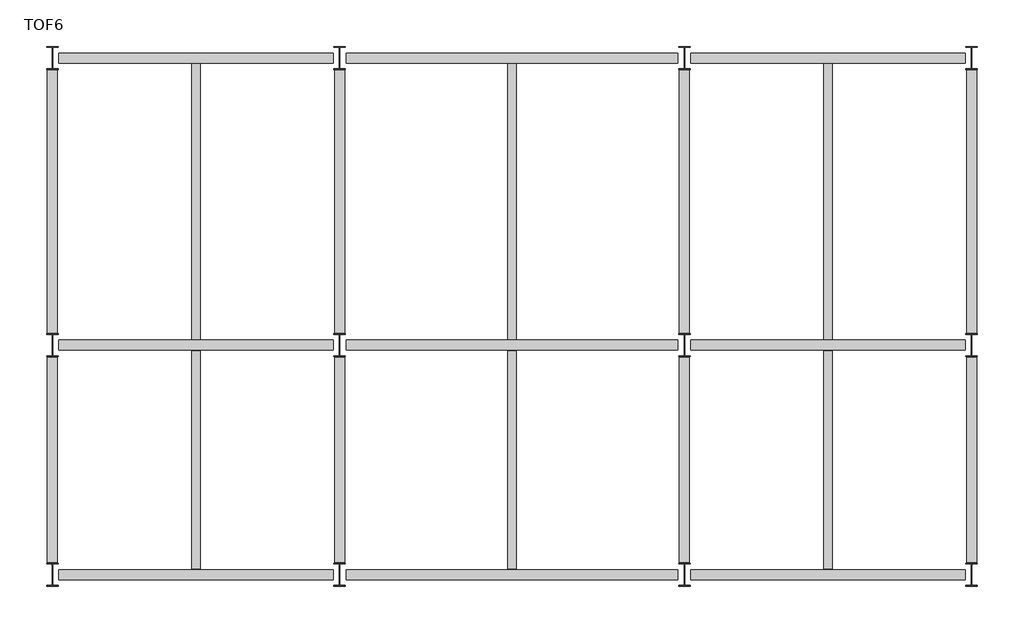
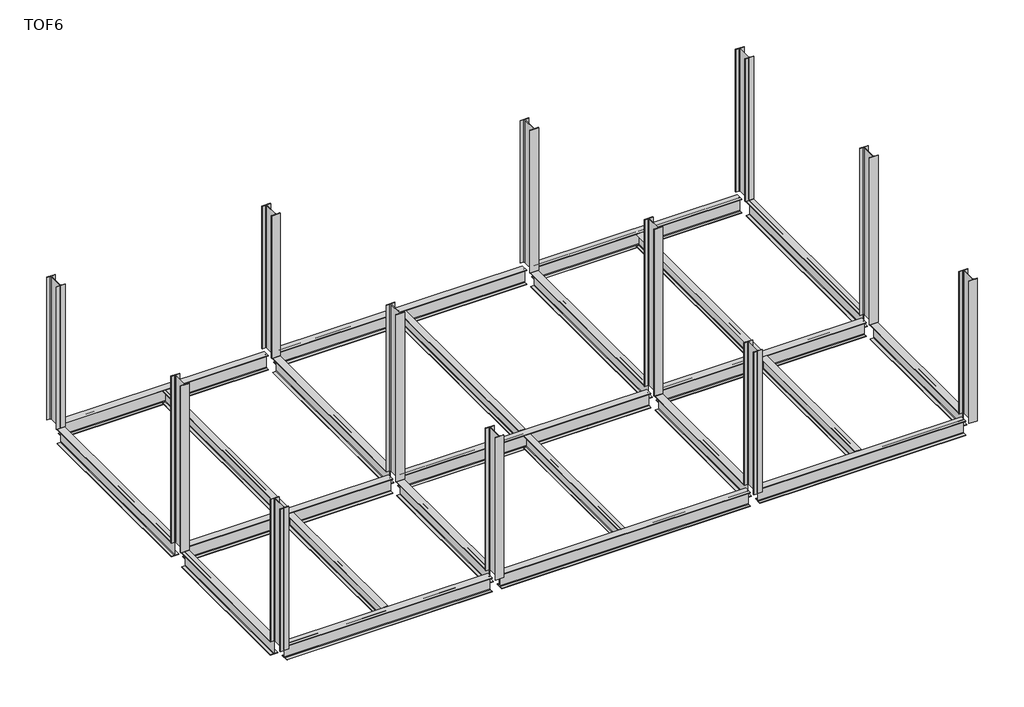
# One storey: 23 beams, 12 columns.
"""IFC4 building model written with IfcOpenShell, lengths in millimetres."""

import ifcopenshell
import ifcopenshell.guid

model = None  # the IFC model being written
_history = None  # IfcOwnerHistory: only IFC2X3 demands one
_inside = {}  # id of a spatial element -> (the spatial element, [elements in it])
_under = {}  # id of a project, library or spatial element -> (it, [spatial elements below it])
_declared = {}  # id of a project -> (the project, [libraries it declares])
_typed = {}  # id of a type object -> (the type object, [elements of that type])
_made_of = {}  # id of a material, layer set ... -> (it, [elements and type objects made of it])


def new_model(schema):
    """Start an empty IFC model of exactly this schema.

    Asked for "IFC4X3", IfcOpenShell would pick the latest addendum, in which some entities
    have other attributes; the version numbers below select the first issue.
    IFC2X3 requires an IfcOwnerHistory on every rooted entity: one is made here for all.
    """
    global model, _history
    if schema == "IFC4X3":
        model = ifcopenshell.file(schema_version=(4, 3, 0, 0))
    else:
        model = ifcopenshell.file(schema=schema)
    _inside.clear()
    _under.clear()
    _declared.clear()
    _typed.clear()
    _made_of.clear()
    _history = None
    if model.schema == "IFC2X3":
        org = make("IfcOrganization", Name="unknown")
        user = make(
            "IfcPersonAndOrganization",
            ThePerson=make("IfcPerson", FamilyName="unknown"),
            TheOrganization=org,
        )
        app = make(
            "IfcApplication",
            ApplicationDeveloper=org,
            Version="unknown",
            ApplicationFullName="unknown",
            ApplicationIdentifier="unknown",
        )
        _history = make(
            "IfcOwnerHistory",
            OwningUser=user,
            OwningApplication=app,
            ChangeAction="ADDED",
            CreationDate=0,
        )
    return model


def make(cls, **values):
    """One entity of the class cls with the attributes given. An attribute that is None is left unset."""
    return model.create_entity(
        cls, **{name: value for name, value in values.items() if value is not None}
    )


def rooted(cls, **values):
    """An entity with a GlobalId (a new one), such as an element, a storey or a relation."""
    return make(cls, GlobalId=ifcopenshell.guid.new(), OwnerHistory=_history, **values)


def si_unit(unit_type, name, prefix=None):
    """IfcSIUnit, for example si_unit("LENGTHUNIT", "METRE", prefix="MILLI")."""
    return make("IfcSIUnit", UnitType=unit_type, Prefix=prefix, Name=name)


def assignment(units):
    """IfcUnitAssignment: the units of a project."""
    return None if units is None else make("IfcUnitAssignment", Units=units)


def point(xyz):
    """IfcCartesianPoint."""
    return None if xyz is None else make("IfcCartesianPoint", Coordinates=xyz)


def direction(xyz):
    """IfcDirection."""
    return None if xyz is None else make("IfcDirection", DirectionRatios=xyz)


def frame(location, z_axis=None, x_axis=None):
    """IfcAxis2Placement3D, a coordinate frame: its origin and axes. An axis left out is left unset."""
    return make(
        "IfcAxis2Placement3D",
        Location=point(location),
        Axis=direction(z_axis),
        RefDirection=direction(x_axis),
    )


def frame_2d(location, x_axis=None):
    """IfcAxis2Placement2D, a coordinate frame in the plane: its origin and x axis."""
    return make(
        "IfcAxis2Placement2D", Location=point(location), RefDirection=direction(x_axis)
    )


def origin():
    """The frame at (0, 0, 0) with its axes left unset."""
    return frame((0.0, 0.0, 0.0))


def place(relative_to, where):
    """IfcLocalPlacement: puts the frame where relative to a parent placement (None: the world)."""
    return make(
        "IfcLocalPlacement", PlacementRelTo=relative_to, RelativePlacement=where
    )


def context(
    kind, dimensions, precision=None, world=None, true_north=None, identifier=None
):
    """IfcGeometricRepresentationContext, for example the 3D "Model" context."""
    return make(
        "IfcGeometricRepresentationContext",
        ContextIdentifier=identifier,
        ContextType=kind,
        CoordinateSpaceDimension=dimensions,
        Precision=precision,
        WorldCoordinateSystem=world,
        TrueNorth=true_north,
    )


def project(units=None, contexts=None):
    """IfcProject with its units and contexts."""
    return rooted(
        "IfcProject",
        Name="project",
        RepresentationContexts=contexts,
        UnitsInContext=assignment(units),
    )


def spatial(cls, under=None, at=None, **own):
    """A site, building, storey or space (cls), placed at a placement, below another one or the project."""
    s = rooted(cls, ObjectPlacement=at, **own)
    if under is not None:
        _under.setdefault(under.id(), (under, []))[1].append(s)
    return s


def polyline(points):
    """IfcPolyline through the points."""
    return make("IfcPolyline", Points=[point(p) for p in points])


def circle_curve(where, radius):
    """IfcCircle in the frame where."""
    return make("IfcCircle", Position=where, Radius=radius)


def trimmed(basis, trim1, trim2, sense, master):
    """IfcTrimmedCurve: the piece of a basis curve between two trims."""
    return make(
        "IfcTrimmedCurve",
        BasisCurve=basis,
        Trim1=trim1,
        Trim2=trim2,
        SenseAgreement=sense,
        MasterRepresentation=master,
    )


def segment(curve, same_sense, transition):
    """IfcCompositeCurveSegment."""
    return make(
        "IfcCompositeCurveSegment",
        Transition=transition,
        SameSense=same_sense,
        ParentCurve=curve,
    )


def composite_curve(segments, self_intersect=None):
    """IfcCompositeCurve: segments joined end to end."""
    return make("IfcCompositeCurve", Segments=segments, SelfIntersect=self_intersect)


def outline(outer, holes=None, kind="AREA"):
    """IfcArbitraryClosedProfileDef: a profile drawn as a closed curve; with holes, ...WithVoids."""
    if holes is None:
        return make("IfcArbitraryClosedProfileDef", ProfileType=kind, OuterCurve=outer)
    return make(
        "IfcArbitraryProfileDefWithVoids",
        ProfileType=kind,
        OuterCurve=outer,
        InnerCurves=holes,
    )


def extrude(swept, where, along, depth):
    """IfcExtrudedAreaSolid: the profile swept, set in the frame where, extruded along a direction by depth."""
    return make(
        "IfcExtrudedAreaSolid",
        SweptArea=swept,
        Position=where,
        ExtrudedDirection=direction(along),
        Depth=depth,
    )


def shape(context_of_items, identifier, shape_type, items):
    """IfcShapeRepresentation: the items that make up one representation, for example the "Body"."""
    return make(
        "IfcShapeRepresentation",
        ContextOfItems=context_of_items,
        RepresentationIdentifier=identifier,
        RepresentationType=shape_type,
        Items=items,
    )


def source(mapping_origin, context_of_items, identifier, shape_type, items):
    """IfcRepresentationMap: a shape defined once, which mapped items show again and again."""
    return make(
        "IfcRepresentationMap",
        MappingOrigin=mapping_origin,
        MappedRepresentation=shape(context_of_items, identifier, shape_type, items),
    )


def transform(
    local_origin,
    x_axis=None,
    y_axis=None,
    z_axis=None,
    scale=None,
    scale2=None,
    scale3=None,
    uniform=True,
):
    """IfcCartesianTransformationOperator3D, or its non-uniform kind. x_axis, y_axis, z_axis: its Axis1, 2, 3."""
    if uniform:
        return make(
            "IfcCartesianTransformationOperator3D",
            Axis1=direction(x_axis),
            Axis2=direction(y_axis),
            LocalOrigin=point(local_origin),
            Scale=scale,
            Axis3=direction(z_axis),
        )
    return make(
        "IfcCartesianTransformationOperator3DnonUniform",
        Axis1=direction(x_axis),
        Axis2=direction(y_axis),
        LocalOrigin=point(local_origin),
        Scale=scale,
        Axis3=direction(z_axis),
        Scale2=scale2,
        Scale3=scale3,
    )


def mapped(mapping_source, mapping_target):
    """IfcMappedItem: shows the shape of a source again, moved by a transform."""
    return make(
        "IfcMappedItem", MappingSource=mapping_source, MappingTarget=mapping_target
    )


def made_of(thing, what):
    """Note that an element or type object is made of a material, layer set ...; save() writes the relation."""
    if what is not None:
        _made_of.setdefault(what.id(), (what, []))[1].append(thing)
    return thing


def element(
    cls,
    number,
    at=None,
    inside=None,
    cuts=None,
    type_object=None,
    material=None,
    context=None,
    identifier="Body",
    shape_type=None,
    held_by="IfcProductDefinitionShape",
    body=None,
    shapes=None,
    **own,
):
    """One element of the class cls, such as IfcWall. Its Tag is "e" and its number.

    at: its placement. inside: the storey or other place that contains it. cuts: it is an
    opening in that element (IfcRelVoidsElement). A single representation is given by context,
    identifier, shape_type and body (its items); several are given by shapes. held_by: the class
    of the entity that holds the representations. save() writes the other relations.
    """
    e = rooted(cls, Tag="e%d" % number, ObjectPlacement=at, **own)
    if body is not None:
        shapes = [shape(context, identifier, shape_type, body)]
    if shapes is not None:
        e.Representation = make(held_by, Representations=shapes)
    if inside is not None:
        _inside.setdefault(inside.id(), (inside, []))[1].append(e)
    if cuts is not None:
        rooted(
            "IfcRelVoidsElement", RelatingBuildingElement=cuts, RelatedOpeningElement=e
        )
    if type_object is not None:
        _typed.setdefault(type_object.id(), (type_object, []))[1].append(e)
    return made_of(e, material)


def aggregate(whole, parts):
    """IfcRelAggregates: a whole, such as a stair, and the parts it consists of."""
    return rooted("IfcRelAggregates", RelatingObject=whole, RelatedObjects=parts)


def save(model, path):
    """Write the relations noted so far, then the file.

    IfcRelAggregates (storeys below a building ...), IfcRelContainedInSpatialStructure (elements
    in a storey), IfcRelDefinesByType, IfcRelAssociatesMaterial and IfcRelDeclares: one each for
    every whole, place, type object, material and project.
    """
    for whole, parts in _under.values():
        aggregate(whole, parts)
    for where, things in _inside.values():
        rooted(
            "IfcRelContainedInSpatialStructure",
            RelatedElements=things,
            RelatingStructure=where,
        )
    for kind, things in _typed.values():
        rooted("IfcRelDefinesByType", RelatedObjects=things, RelatingType=kind)
    for what, things in _made_of.values():
        rooted("IfcRelAssociatesMaterial", RelatedObjects=things, RelatingMaterial=what)
    for by, libraries in _declared.values():
        rooted("IfcRelDeclares", RelatingContext=by, RelatedDefinitions=libraries)
    model.write(path)


def beam_edbab3fa(model_context):
    return source(origin(), model_context, "Body", "SweptSolid", [
        extrude(outline(composite_curve([segment(polyline([(75.0, -141.0), (75.0, -150.0), (-75.0, -150.0), (-75.0, -141.0), (-16.25, -141.0)]), True, "CONTINUOUS"), segment(trimmed(circle_curve(frame_2d((-16.25, -128.0)), 13.0), [point((-16.25, -141.0))], [point((-3.25, -128.0))], True, "CARTESIAN"), True, "CONTINUOUS"), segment(polyline([(-3.25, -128.0), (-3.25, 128.0)]), True, "CONTINUOUS"), segment(trimmed(circle_curve(frame_2d((-16.25, 128.0)), 13.0), [point((-3.25, 128.0))], [point((-16.25, 141.0))], True, "CARTESIAN"), True, "CONTINUOUS"), segment(polyline([(-16.25, 141.0), (-75.0, 141.0), (-75.0, 150.0), (75.0, 150.0), (75.0, 141.0), (16.25, 141.0)]), True, "CONTINUOUS"), segment(trimmed(circle_curve(frame_2d((16.25, 128.0)), 13.0), [point((16.25, 141.0))], [point((3.25, 128.0))], True, "CARTESIAN"), True, "CONTINUOUS"), segment(polyline([(3.25, 128.0), (3.25, -128.0)]), True, "CONTINUOUS"), segment(trimmed(circle_curve(frame_2d((16.25, -128.0)), 13.0), [point((3.25, -128.0))], [point((16.25, -141.0))], True, "CARTESIAN"), True, "CONTINUOUS"), segment(polyline([(16.25, -141.0), (75.0, -141.0)]), True, "CONTINUOUS")], self_intersect=False)), frame((-1899.8, 0.0, 0.0), z_axis=(1.0, 0.0, 0.0), x_axis=(0.0, 1.0, 0.0)), (0.0, 0.0, 1.0), 3799.6),
    ])


def beam_c00964ff(model_context):
    return source(origin(), model_context, "Body", "SweptSolid", [
        extrude(outline(composite_curve([segment(polyline([(75.0, -141.0), (75.0, -150.0), (-75.0, -150.0), (-75.0, -141.0), (-16.25, -141.0)]), True, "CONTINUOUS"), segment(trimmed(circle_curve(frame_2d((-16.25, -128.0)), 13.0), [point((-16.25, -141.0))], [point((-3.25, -128.0))], True, "CARTESIAN"), True, "CONTINUOUS"), segment(polyline([(-3.25, -128.0), (-3.25, 128.0)]), True, "CONTINUOUS"), segment(trimmed(circle_curve(frame_2d((-16.25, 128.0)), 13.0), [point((-3.25, 128.0))], [point((-16.25, 141.0))], True, "CARTESIAN"), True, "CONTINUOUS"), segment(polyline([(-16.25, 141.0), (-75.0, 141.0), (-75.0, 150.0), (75.0, 150.0), (75.0, 141.0), (16.25, 141.0)]), True, "CONTINUOUS"), segment(trimmed(circle_curve(frame_2d((16.25, 128.0)), 13.0), [point((16.25, 141.0))], [point((3.25, 128.0))], True, "CARTESIAN"), True, "CONTINUOUS"), segment(polyline([(3.25, 128.0), (3.25, -128.0)]), True, "CONTINUOUS"), segment(trimmed(circle_curve(frame_2d((16.25, -128.0)), 13.0), [point((3.25, -128.0))], [point((16.25, -141.0))], True, "CARTESIAN"), True, "CONTINUOUS"), segment(polyline([(16.25, -141.0), (75.0, -141.0)]), True, "CONTINUOUS")], self_intersect=False)), frame((-2399.8, 0.0, 0.0), z_axis=(1.0, 0.0, 0.0), x_axis=(0.0, 1.0, 0.0)), (0.0, 0.0, 1.0), 4799.6),
    ])


def beam_74d50635(model_context):
    return source(origin(), model_context, "Body", "SweptSolid", [
        extrude(outline(composite_curve([segment(polyline([(87.5, -164.0), (87.5, -175.0), (-87.5, -175.0), (-87.5, -164.0), (-17.5, -164.0)]), True, "CONTINUOUS"), segment(trimmed(circle_curve(frame_2d((-17.5, -150.0)), 14.0), [point((-17.5, -164.0))], [point((-3.5, -150.0))], True, "CARTESIAN"), True, "CONTINUOUS"), segment(polyline([(-3.5, -150.0), (-3.5, 150.0)]), True, "CONTINUOUS"), segment(trimmed(circle_curve(frame_2d((-17.5, 150.0)), 14.0), [point((-3.5, 150.0))], [point((-17.5, 164.0))], True, "CARTESIAN"), True, "CONTINUOUS"), segment(polyline([(-17.5, 164.0), (-87.5, 164.0), (-87.5, 175.0), (87.5, 175.0), (87.5, 164.0), (17.5, 164.0)]), True, "CONTINUOUS"), segment(trimmed(circle_curve(frame_2d((17.5, 150.0)), 14.0), [point((17.5, 164.0))], [point((3.5, 150.0))], True, "CARTESIAN"), True, "CONTINUOUS"), segment(polyline([(3.5, 150.0), (3.5, -150.0)]), True, "CONTINUOUS"), segment(trimmed(circle_curve(frame_2d((17.5, -150.0)), 14.0), [point((3.5, -150.0))], [point((17.5, -164.0))], True, "CARTESIAN"), True, "CONTINUOUS"), segment(polyline([(17.5, -164.0), (87.5, -164.0)]), True, "CONTINUOUS")], self_intersect=False)), frame((-2387.3, 0.0, 0.0), z_axis=(1.0, 0.0, 0.0), x_axis=(0.0, 1.0, 0.0)), (0.0, 0.0, 1.0), 4774.6),
    ])


def beam_3a5a8fac(model_context):
    return source(origin(), model_context, "Body", "SweptSolid", [
        extrude(outline(composite_curve([segment(polyline([(87.5, -164.0), (87.5, -175.0), (-87.5, -175.0), (-87.5, -164.0), (-17.5, -164.0)]), True, "CONTINUOUS"), segment(trimmed(circle_curve(frame_2d((-17.5, -150.0)), 14.0), [point((-17.5, -164.0))], [point((-3.5, -150.0))], True, "CARTESIAN"), True, "CONTINUOUS"), segment(polyline([(-3.5, -150.0), (-3.5, 150.0)]), True, "CONTINUOUS"), segment(trimmed(circle_curve(frame_2d((-17.5, 150.0)), 14.0), [point((-3.5, 150.0))], [point((-17.5, 164.0))], True, "CARTESIAN"), True, "CONTINUOUS"), segment(polyline([(-17.5, 164.0), (-87.5, 164.0), (-87.5, 175.0), (87.5, 175.0), (87.5, 164.0), (17.5, 164.0)]), True, "CONTINUOUS"), segment(trimmed(circle_curve(frame_2d((17.5, 150.0)), 14.0), [point((17.5, 164.0))], [point((3.5, 150.0))], True, "CARTESIAN"), True, "CONTINUOUS"), segment(polyline([(3.5, 150.0), (3.5, -150.0)]), True, "CONTINUOUS"), segment(trimmed(circle_curve(frame_2d((17.5, -150.0)), 14.0), [point((3.5, -150.0))], [point((17.5, -164.0))], True, "CARTESIAN"), True, "CONTINUOUS"), segment(polyline([(17.5, -164.0), (87.5, -164.0)]), True, "CONTINUOUS")], self_intersect=False)), frame((-2887.3, 0.0, 0.0), z_axis=(1.0, 0.0, 0.0), x_axis=(0.0, 1.0, 0.0)), (0.0, 0.0, 1.0), 5774.6),
    ])


def beam_edcef29c(model_context):
    return source(origin(), model_context, "Body", "SweptSolid", [
        extrude(outline(composite_curve([segment(polyline([(87.5, -164.0), (87.5, -175.0), (-87.5, -175.0), (-87.5, -164.0), (-17.5, -164.0)]), True, "CONTINUOUS"), segment(trimmed(circle_curve(frame_2d((-17.5, -150.0)), 14.0), [point((-17.5, -164.0))], [point((-3.5, -150.0))], True, "CARTESIAN"), True, "CONTINUOUS"), segment(polyline([(-3.5, -150.0), (-3.5, 150.0)]), True, "CONTINUOUS"), segment(trimmed(circle_curve(frame_2d((-17.5, 150.0)), 14.0), [point((-3.5, 150.0))], [point((-17.5, 164.0))], True, "CARTESIAN"), True, "CONTINUOUS"), segment(polyline([(-17.5, 164.0), (-87.5, 164.0), (-87.5, 175.0), (87.5, 175.0), (87.5, 164.0), (17.5, 164.0)]), True, "CONTINUOUS"), segment(trimmed(circle_curve(frame_2d((17.5, 150.0)), 14.0), [point((17.5, 164.0))], [point((3.5, 150.0))], True, "CARTESIAN"), True, "CONTINUOUS"), segment(polyline([(3.5, 150.0), (3.5, -150.0)]), True, "CONTINUOUS"), segment(trimmed(circle_curve(frame_2d((17.5, -150.0)), 14.0), [point((3.5, -150.0))], [point((17.5, -164.0))], True, "CARTESIAN"), True, "CONTINUOUS"), segment(polyline([(17.5, -164.0), (87.5, -164.0)]), True, "CONTINUOUS")], self_intersect=False)), frame((-1787.3, 0.0, 0.0), z_axis=(1.0, 0.0, 0.0), x_axis=(0.0, 1.0, 0.0)), (0.0, 0.0, 1.0), 3574.6),
    ])


def beam_68894c75(model_context):
    return source(origin(), model_context, "Body", "SweptSolid", [
        extrude(outline(composite_curve([segment(polyline([(87.5, -164.0), (87.5, -175.0), (-87.5, -175.0), (-87.5, -164.0), (-17.5, -164.0)]), True, "CONTINUOUS"), segment(trimmed(circle_curve(frame_2d((-17.5, -150.0)), 14.0), [point((-17.5, -164.0))], [point((-3.5, -150.0))], True, "CARTESIAN"), True, "CONTINUOUS"), segment(polyline([(-3.5, -150.0), (-3.5, 150.0)]), True, "CONTINUOUS"), segment(trimmed(circle_curve(frame_2d((-17.5, 150.0)), 14.0), [point((-3.5, 150.0))], [point((-17.5, 164.0))], True, "CARTESIAN"), True, "CONTINUOUS"), segment(polyline([(-17.5, 164.0), (-87.5, 164.0), (-87.5, 175.0), (87.5, 175.0), (87.5, 164.0), (17.5, 164.0)]), True, "CONTINUOUS"), segment(trimmed(circle_curve(frame_2d((17.5, 150.0)), 14.0), [point((17.5, 164.0))], [point((3.5, 150.0))], True, "CARTESIAN"), True, "CONTINUOUS"), segment(polyline([(3.5, 150.0), (3.5, -150.0)]), True, "CONTINUOUS"), segment(trimmed(circle_curve(frame_2d((17.5, -150.0)), 14.0), [point((3.5, -150.0))], [point((17.5, -164.0))], True, "CARTESIAN"), True, "CONTINUOUS"), segment(polyline([(17.5, -164.0), (87.5, -164.0)]), True, "CONTINUOUS")], self_intersect=False)), frame((-2287.3, 0.0, 0.0), z_axis=(1.0, 0.0, 0.0), x_axis=(0.0, 1.0, 0.0)), (0.0, 0.0, 1.0), 4574.6),
    ])


model = new_model("IFC4")

# Units and contexts
model_context = context("Model", 3, world=origin())
ifc_project = project(units=[si_unit("LENGTHUNIT", "METRE", prefix="MILLI")], contexts=[model_context])

# Site, building, storey
site = spatial("IfcSite", under=ifc_project)
building = spatial("IfcBuilding", under=site)
storey = spatial("IfcBuildingStorey", under=building, Name="TOF6", Elevation=9000.0)

# Beams
placement = place(None, origin())
beam_shape = beam_edbab3fa(model_context)
element("IfcBeam", 1, ObjectType="0912_Steel Framing_H-KSD3502 : H_SB_AR_S02_H-300x150x6.5x9_Stair", at=placement, inside=storey, context=model_context, shape_type="MappedRepresentation", body=[
    mapped(beam_shape, transform((2500.0, 2000.0, 8850.0), x_axis=(0.0, 1.0, 0.0), y_axis=(-1.0, 0.0, 0.0), z_axis=(0.0, 0.0, 1.0))),
])
element("IfcBeam", 2, ObjectType="0912_Steel Framing_H-KSD3502 : H_SB_AR_S02_H-300x150x6.5x9_Stair", at=placement, inside=storey, context=model_context, shape_type="MappedRepresentation", body=[
    mapped(beam_shape, transform((8000.0, 2000.0, 8850.0), x_axis=(0.0, 1.0, 0.0), y_axis=(-1.0, 0.0, 0.0), z_axis=(0.0, 0.0, 1.0))),
])
element("IfcBeam", 3, ObjectType="0912_Steel Framing_H-KSD3502 : H_SB_AR_S02_H-300x150x6.5x9_Stair", at=placement, inside=storey, context=model_context, shape_type="MappedRepresentation", body=[
    mapped(beam_shape, transform((13500.0, 2000.0, 8850.0), x_axis=(0.0, 1.0, 0.0), y_axis=(-1.0, 0.0, 0.0), z_axis=(0.0, 0.0, 1.0))),
])
beam_2_shape = beam_c00964ff(model_context)
element("IfcBeam", 4, ObjectType="0912_Steel Framing_H-KSD3502 : H_SB_AR_S02_H-300x150x6.5x9_Stair", at=placement, inside=storey, context=model_context, shape_type="MappedRepresentation", body=[
    mapped(beam_2_shape, transform((2500.0, 6500.0, 8850.0), x_axis=(0.0, 1.0, 0.0), y_axis=(-1.0, 0.0, 0.0), z_axis=(0.0, 0.0, 1.0))),
])
element("IfcBeam", 5, ObjectType="0912_Steel Framing_H-KSD3502 : H_SB_AR_S02_H-300x150x6.5x9_Stair", at=placement, inside=storey, context=model_context, shape_type="MappedRepresentation", body=[
    mapped(beam_2_shape, transform((8000.0, 6500.0, 8850.0), x_axis=(0.0, 1.0, 0.0), y_axis=(-1.0, 0.0, 0.0), z_axis=(0.0, 0.0, 1.0))),
])
element("IfcBeam", 6, ObjectType="0912_Steel Framing_H-KSD3502 : H_SB_AR_S02_H-300x150x6.5x9_Stair", at=placement, inside=storey, context=model_context, shape_type="MappedRepresentation", body=[
    mapped(beam_2_shape, transform((13500.0, 6500.0, 8850.0), x_axis=(0.0, 1.0, 0.0), y_axis=(-1.0, 0.0, 0.0), z_axis=(0.0, 0.0, 1.0))),
])
beam_3_shape = beam_74d50635(model_context)
element("IfcBeam", 7, ObjectType="0912_Steel Framing_H-KSD3502 : H_SB_AR_S02_H-350x175x7x11_Platform", at=placement, inside=storey, context=model_context, shape_type="MappedRepresentation", body=[
    mapped(beam_3_shape, transform((2500.0, 0.0, 8825.0), x_axis=(1.0, 0.0, 0.0), y_axis=(0.0, 1.0, 0.0), z_axis=(0.0, 0.0, 1.0))),
])
element("IfcBeam", 8, ObjectType="0912_Steel Framing_H-KSD3502 : H_SB_AR_S02_H-350x175x7x11_Platform", at=placement, inside=storey, context=model_context, shape_type="MappedRepresentation", body=[
    mapped(beam_3_shape, transform((13500.0, 0.0, 8825.0), x_axis=(1.0, 0.0, 0.0), y_axis=(0.0, 1.0, 0.0), z_axis=(0.0, 0.0, 1.0))),
])
element("IfcBeam", 9, ObjectType="0912_Steel Framing_H-KSD3502 : H_SB_AR_S02_H-350x175x7x11_Platform", at=placement, inside=storey, context=model_context, shape_type="MappedRepresentation", body=[
    mapped(beam_3_shape, transform((2500.0, 4000.0, 8825.0), x_axis=(1.0, 0.0, 0.0), y_axis=(0.0, 1.0, 0.0), z_axis=(0.0, 0.0, 1.0))),
])
element("IfcBeam", 10, ObjectType="0912_Steel Framing_H-KSD3502 : H_SB_AR_S02_H-350x175x7x11_Platform", at=placement, inside=storey, context=model_context, shape_type="MappedRepresentation", body=[
    mapped(beam_3_shape, transform((13500.0, 4000.0, 8825.0), x_axis=(1.0, 0.0, 0.0), y_axis=(0.0, 1.0, 0.0), z_axis=(0.0, 0.0, 1.0))),
])
element("IfcBeam", 11, ObjectType="0912_Steel Framing_H-KSD3502 : H_SB_AR_S02_H-350x175x7x11_Platform", at=placement, inside=storey, context=model_context, shape_type="MappedRepresentation", body=[
    mapped(beam_3_shape, transform((2500.0, 9000.0, 8825.0), x_axis=(1.0, 0.0, 0.0), y_axis=(0.0, 1.0, 0.0), z_axis=(0.0, 0.0, 1.0))),
])
element("IfcBeam", 12, ObjectType="0912_Steel Framing_H-KSD3502 : H_SB_AR_S02_H-350x175x7x11_Platform", at=placement, inside=storey, context=model_context, shape_type="MappedRepresentation", body=[
    mapped(beam_3_shape, transform((13500.0, 9000.0, 8825.0), x_axis=(1.0, 0.0, 0.0), y_axis=(0.0, 1.0, 0.0), z_axis=(0.0, 0.0, 1.0))),
])
beam_4_shape = beam_3a5a8fac(model_context)
element("IfcBeam", 13, ObjectType="0912_Steel Framing_H-KSD3502 : H_SB_AR_S02_H-350x175x7x11_Platform", at=placement, inside=storey, context=model_context, shape_type="MappedRepresentation", body=[
    mapped(beam_4_shape, transform((8000.0, 0.0, 8825.0), x_axis=(1.0, 0.0, 0.0), y_axis=(0.0, 1.0, 0.0), z_axis=(0.0, 0.0, 1.0))),
])
element("IfcBeam", 14, ObjectType="0912_Steel Framing_H-KSD3502 : H_SB_AR_S02_H-350x175x7x11_Platform", at=placement, inside=storey, context=model_context, shape_type="MappedRepresentation", body=[
    mapped(beam_4_shape, transform((8000.0, 4000.0, 8825.0), x_axis=(1.0, 0.0, 0.0), y_axis=(0.0, 1.0, 0.0), z_axis=(0.0, 0.0, 1.0))),
])
element("IfcBeam", 15, ObjectType="0912_Steel Framing_H-KSD3502 : H_SB_AR_S02_H-350x175x7x11_Platform", at=placement, inside=storey, context=model_context, shape_type="MappedRepresentation", body=[
    mapped(beam_4_shape, transform((8000.0, 9000.0, 8825.0), x_axis=(1.0, 0.0, 0.0), y_axis=(0.0, 1.0, 0.0), z_axis=(0.0, 0.0, 1.0))),
])
beam_5_shape = beam_edcef29c(model_context)
element("IfcBeam", 16, ObjectType="0912_Steel Framing_H-KSD3502 : H_SB_AR_S02_H-350x175x7x11_Platform", at=placement, inside=storey, context=model_context, shape_type="MappedRepresentation", body=[
    mapped(beam_5_shape, transform((0.0, 2000.0, 8825.0), x_axis=(0.0, 1.0, 0.0), y_axis=(-1.0, 0.0, 0.0), z_axis=(0.0, 0.0, 1.0))),
])
element("IfcBeam", 17, ObjectType="0912_Steel Framing_H-KSD3502 : H_SB_AR_S02_H-350x175x7x11_Platform", at=placement, inside=storey, context=model_context, shape_type="MappedRepresentation", body=[
    mapped(beam_5_shape, transform((5000.0, 2000.0, 8825.0), x_axis=(0.0, 1.0, 0.0), y_axis=(-1.0, 0.0, 0.0), z_axis=(0.0, 0.0, 1.0))),
])
element("IfcBeam", 18, ObjectType="0912_Steel Framing_H-KSD3502 : H_SB_AR_S02_H-350x175x7x11_Platform", at=placement, inside=storey, context=model_context, shape_type="MappedRepresentation", body=[
    mapped(beam_5_shape, transform((11000.0, 2000.0, 8825.0), x_axis=(0.0, 1.0, 0.0), y_axis=(-1.0, 0.0, 0.0), z_axis=(0.0, 0.0, 1.0))),
])
element("IfcBeam", 19, ObjectType="0912_Steel Framing_H-KSD3502 : H_SB_AR_S02_H-350x175x7x11_Platform", at=placement, inside=storey, context=model_context, shape_type="MappedRepresentation", body=[
    mapped(beam_5_shape, transform((16000.0, 2000.0, 8825.0), x_axis=(0.0, 1.0, 0.0), y_axis=(-1.0, 0.0, 0.0), z_axis=(0.0, 0.0, 1.0))),
])
beam_6_shape = beam_68894c75(model_context)
element("IfcBeam", 20, ObjectType="0912_Steel Framing_H-KSD3502 : H_SB_AR_S02_H-350x175x7x11_Platform", at=placement, inside=storey, context=model_context, shape_type="MappedRepresentation", body=[
    mapped(beam_6_shape, transform((0.0, 6500.0, 8825.0), x_axis=(0.0, 1.0, 0.0), y_axis=(-1.0, 0.0, 0.0), z_axis=(0.0, 0.0, 1.0))),
])
element("IfcBeam", 21, ObjectType="0912_Steel Framing_H-KSD3502 : H_SB_AR_S02_H-350x175x7x11_Platform", at=placement, inside=storey, context=model_context, shape_type="MappedRepresentation", body=[
    mapped(beam_6_shape, transform((5000.0, 6500.0, 8825.0), x_axis=(0.0, 1.0, 0.0), y_axis=(-1.0, 0.0, 0.0), z_axis=(0.0, 0.0, 1.0))),
])
element("IfcBeam", 22, ObjectType="0912_Steel Framing_H-KSD3502 : H_SB_AR_S02_H-350x175x7x11_Platform", at=placement, inside=storey, context=model_context, shape_type="MappedRepresentation", body=[
    mapped(beam_6_shape, transform((11000.0, 6500.0, 8825.0), x_axis=(0.0, 1.0, 0.0), y_axis=(-1.0, 0.0, 0.0), z_axis=(0.0, 0.0, 1.0))),
])
element("IfcBeam", 23, ObjectType="0912_Steel Framing_H-KSD3502 : H_SB_AR_S02_H-350x175x7x11_Platform", at=placement, inside=storey, context=model_context, shape_type="MappedRepresentation", body=[
    mapped(beam_6_shape, transform((16000.0, 6500.0, 8825.0), x_axis=(0.0, 1.0, 0.0), y_axis=(-1.0, 0.0, 0.0), z_axis=(0.0, 0.0, 1.0))),
])

# Columns
element("IfcColumn", 24, ObjectType="Steel Column_H_KSD3502 : H_SC_AR_S01_H-400x200x8x13", at=placement, inside=storey, context=model_context, shape_type="SweptSolid", body=[
    extrude(outline(composite_curve([segment(polyline([(100.0, 200.0), (100.0, 187.0), (20.0, 187.0)]), True, "CONTINUOUS"), segment(trimmed(circle_curve(frame_2d((20.0, 171.0)), 16.0), [point((20.0, 187.0))], [point((4.0, 171.0))], True, "CARTESIAN"), True, "CONTINUOUS"), segment(polyline([(4.0, 171.0), (4.0, -171.0)]), True, "CONTINUOUS"), segment(trimmed(circle_curve(frame_2d((20.0, -171.0)), 16.0), [point((4.0, -171.0))], [point((20.0, -187.0))], True, "CARTESIAN"), True, "CONTINUOUS"), segment(polyline([(20.0, -187.0), (100.0, -187.0), (100.0, -200.0), (-100.0, -200.0), (-100.0, -187.0), (-20.0, -187.0)]), True, "CONTINUOUS"), segment(trimmed(circle_curve(frame_2d((-20.0, -171.0)), 16.0), [point((-20.0, -187.0))], [point((-4.0, -171.0))], True, "CARTESIAN"), True, "CONTINUOUS"), segment(polyline([(-4.0, -171.0), (-4.0, 171.0)]), True, "CONTINUOUS"), segment(trimmed(circle_curve(frame_2d((-20.0, 171.0)), 16.0), [point((-4.0, 171.0))], [point((-20.0, 187.0))], True, "CARTESIAN"), True, "CONTINUOUS"), segment(polyline([(-20.0, 187.0), (-100.0, 187.0), (-100.0, 200.0), (100.0, 200.0)]), True, "CONTINUOUS")], self_intersect=False)), frame((0.0, 0.0, 9000.0), z_axis=(0.0, 0.0, 1.0), x_axis=(1.0, 0.0, 0.0)), (0.0, 0.0, 1.0), 3500.0),
])
element("IfcColumn", 25, ObjectType="Steel Column_H_KSD3502 : H_SC_AR_S01_H-400x200x8x13", at=placement, inside=storey, context=model_context, shape_type="SweptSolid", body=[
    extrude(outline(composite_curve([segment(polyline([(5100.0, 200.0), (5100.0, 187.0), (5020.0, 187.0)]), True, "CONTINUOUS"), segment(trimmed(circle_curve(frame_2d((5020.0, 171.0)), 16.0), [point((5020.0, 187.0))], [point((5004.0, 171.0))], True, "CARTESIAN"), True, "CONTINUOUS"), segment(polyline([(5004.0, 171.0), (5004.0, -171.0)]), True, "CONTINUOUS"), segment(trimmed(circle_curve(frame_2d((5020.0, -171.0)), 16.0), [point((5004.0, -171.0))], [point((5020.0, -187.0))], True, "CARTESIAN"), True, "CONTINUOUS"), segment(polyline([(5020.0, -187.0), (5100.0, -187.0), (5100.0, -200.0), (4900.0, -200.0), (4900.0, -187.0), (4980.0, -187.0)]), True, "CONTINUOUS"), segment(trimmed(circle_curve(frame_2d((4980.0, -171.0)), 16.0), [point((4980.0, -187.0))], [point((4996.0, -171.0))], True, "CARTESIAN"), True, "CONTINUOUS"), segment(polyline([(4996.0, -171.0), (4996.0, 171.0)]), True, "CONTINUOUS"), segment(trimmed(circle_curve(frame_2d((4980.0, 171.0)), 16.0), [point((4996.0, 171.0))], [point((4980.0, 187.0))], True, "CARTESIAN"), True, "CONTINUOUS"), segment(polyline([(4980.0, 187.0), (4900.0, 187.0), (4900.0, 200.0), (5100.0, 200.0)]), True, "CONTINUOUS")], self_intersect=False)), frame((0.0, 0.0, 9000.0), z_axis=(0.0, 0.0, 1.0), x_axis=(1.0, 0.0, 0.0)), (0.0, 0.0, 1.0), 3500.0),
])
element("IfcColumn", 26, ObjectType="Steel Column_H_KSD3502 : H_SC_AR_S01_H-400x200x8x13", at=placement, inside=storey, context=model_context, shape_type="SweptSolid", body=[
    extrude(outline(composite_curve([segment(polyline([(11100.0, 200.0), (11100.0, 187.0), (11020.0, 187.0)]), True, "CONTINUOUS"), segment(trimmed(circle_curve(frame_2d((11020.0, 171.0)), 16.0), [point((11020.0, 187.0))], [point((11004.0, 171.0))], True, "CARTESIAN"), True, "CONTINUOUS"), segment(polyline([(11004.0, 171.0), (11004.0, -171.0)]), True, "CONTINUOUS"), segment(trimmed(circle_curve(frame_2d((11020.0, -171.0)), 16.0), [point((11004.0, -171.0))], [point((11020.0, -187.0))], True, "CARTESIAN"), True, "CONTINUOUS"), segment(polyline([(11020.0, -187.0), (11100.0, -187.0), (11100.0, -200.0), (10900.0, -200.0), (10900.0, -187.0), (10980.0, -187.0)]), True, "CONTINUOUS"), segment(trimmed(circle_curve(frame_2d((10980.0, -171.0)), 16.0), [point((10980.0, -187.0))], [point((10996.0, -171.0))], True, "CARTESIAN"), True, "CONTINUOUS"), segment(polyline([(10996.0, -171.0), (10996.0, 171.0)]), True, "CONTINUOUS"), segment(trimmed(circle_curve(frame_2d((10980.0, 171.0)), 16.0), [point((10996.0, 171.0))], [point((10980.0, 187.0))], True, "CARTESIAN"), True, "CONTINUOUS"), segment(polyline([(10980.0, 187.0), (10900.0, 187.0), (10900.0, 200.0), (11100.0, 200.0)]), True, "CONTINUOUS")], self_intersect=False)), frame((0.0, 0.0, 9000.0), z_axis=(0.0, 0.0, 1.0), x_axis=(1.0, 0.0, 0.0)), (0.0, 0.0, 1.0), 3500.0),
])
element("IfcColumn", 27, ObjectType="Steel Column_H_KSD3502 : H_SC_AR_S01_H-400x200x8x13", at=placement, inside=storey, context=model_context, shape_type="SweptSolid", body=[
    extrude(outline(composite_curve([segment(polyline([(16100.0, 200.0), (16100.0, 187.0), (16020.0, 187.0)]), True, "CONTINUOUS"), segment(trimmed(circle_curve(frame_2d((16020.0, 171.0)), 16.0), [point((16020.0, 187.0))], [point((16004.0, 171.0))], True, "CARTESIAN"), True, "CONTINUOUS"), segment(polyline([(16004.0, 171.0), (16004.0, -171.0)]), True, "CONTINUOUS"), segment(trimmed(circle_curve(frame_2d((16020.0, -171.0)), 16.0), [point((16004.0, -171.0))], [point((16020.0, -187.0))], True, "CARTESIAN"), True, "CONTINUOUS"), segment(polyline([(16020.0, -187.0), (16100.0, -187.0), (16100.0, -200.0), (15900.0, -200.0), (15900.0, -187.0), (15980.0, -187.0)]), True, "CONTINUOUS"), segment(trimmed(circle_curve(frame_2d((15980.0, -171.0)), 16.0), [point((15980.0, -187.0))], [point((15996.0, -171.0))], True, "CARTESIAN"), True, "CONTINUOUS"), segment(polyline([(15996.0, -171.0), (15996.0, 171.0)]), True, "CONTINUOUS"), segment(trimmed(circle_curve(frame_2d((15980.0, 171.0)), 16.0), [point((15996.0, 171.0))], [point((15980.0, 187.0))], True, "CARTESIAN"), True, "CONTINUOUS"), segment(polyline([(15980.0, 187.0), (15900.0, 187.0), (15900.0, 200.0), (16100.0, 200.0)]), True, "CONTINUOUS")], self_intersect=False)), frame((0.0, 0.0, 9000.0), z_axis=(0.0, 0.0, 1.0), x_axis=(1.0, 0.0, 0.0)), (0.0, 0.0, 1.0), 3500.0),
])
element("IfcColumn", 28, ObjectType="Steel Column_H_KSD3502 : H_SC_AR_S01_H-400x200x8x13", at=placement, inside=storey, context=model_context, shape_type="SweptSolid", body=[
    extrude(outline(composite_curve([segment(polyline([(100.0, 4200.0), (100.0, 4187.0), (20.0, 4187.0)]), True, "CONTINUOUS"), segment(trimmed(circle_curve(frame_2d((20.0, 4171.0)), 16.0), [point((20.0, 4187.0))], [point((4.0, 4171.0))], True, "CARTESIAN"), True, "CONTINUOUS"), segment(polyline([(4.0, 4171.0), (4.0, 3829.0)]), True, "CONTINUOUS"), segment(trimmed(circle_curve(frame_2d((20.0, 3829.0)), 16.0), [point((4.0, 3829.0))], [point((20.0, 3813.0))], True, "CARTESIAN"), True, "CONTINUOUS"), segment(polyline([(20.0, 3813.0), (100.0, 3813.0), (100.0, 3800.0), (-100.0, 3800.0), (-100.0, 3813.0), (-20.0, 3813.0)]), True, "CONTINUOUS"), segment(trimmed(circle_curve(frame_2d((-20.0, 3829.0)), 16.0), [point((-20.0, 3813.0))], [point((-4.0, 3829.0))], True, "CARTESIAN"), True, "CONTINUOUS"), segment(polyline([(-4.0, 3829.0), (-4.0, 4171.0)]), True, "CONTINUOUS"), segment(trimmed(circle_curve(frame_2d((-20.0, 4171.0)), 16.0), [point((-4.0, 4171.0))], [point((-20.0, 4187.0))], True, "CARTESIAN"), True, "CONTINUOUS"), segment(polyline([(-20.0, 4187.0), (-100.0, 4187.0), (-100.0, 4200.0), (100.0, 4200.0)]), True, "CONTINUOUS")], self_intersect=False)), frame((0.0, 0.0, 9000.0), z_axis=(0.0, 0.0, 1.0), x_axis=(1.0, 0.0, 0.0)), (0.0, 0.0, 1.0), 4100.0),
])
element("IfcColumn", 29, ObjectType="Steel Column_H_KSD3502 : H_SC_AR_S01_H-400x200x8x13", at=placement, inside=storey, context=model_context, shape_type="SweptSolid", body=[
    extrude(outline(composite_curve([segment(polyline([(5100.0, 4200.0), (5100.0, 4187.0), (5020.0, 4187.0)]), True, "CONTINUOUS"), segment(trimmed(circle_curve(frame_2d((5020.0, 4171.0)), 16.0), [point((5020.0, 4187.0))], [point((5004.0, 4171.0))], True, "CARTESIAN"), True, "CONTINUOUS"), segment(polyline([(5004.0, 4171.0), (5004.0, 3829.0)]), True, "CONTINUOUS"), segment(trimmed(circle_curve(frame_2d((5020.0, 3829.0)), 16.0), [point((5004.0, 3829.0))], [point((5020.0, 3813.0))], True, "CARTESIAN"), True, "CONTINUOUS"), segment(polyline([(5020.0, 3813.0), (5100.0, 3813.0), (5100.0, 3800.0), (4900.0, 3800.0), (4900.0, 3813.0), (4980.0, 3813.0)]), True, "CONTINUOUS"), segment(trimmed(circle_curve(frame_2d((4980.0, 3829.0)), 16.0), [point((4980.0, 3813.0))], [point((4996.0, 3829.0))], True, "CARTESIAN"), True, "CONTINUOUS"), segment(polyline([(4996.0, 3829.0), (4996.0, 4171.0)]), True, "CONTINUOUS"), segment(trimmed(circle_curve(frame_2d((4980.0, 4171.0)), 16.0), [point((4996.0, 4171.0))], [point((4980.0, 4187.0))], True, "CARTESIAN"), True, "CONTINUOUS"), segment(polyline([(4980.0, 4187.0), (4900.0, 4187.0), (4900.0, 4200.0), (5100.0, 4200.0)]), True, "CONTINUOUS")], self_intersect=False)), frame((0.0, 0.0, 9000.0), z_axis=(0.0, 0.0, 1.0), x_axis=(1.0, 0.0, 0.0)), (0.0, 0.0, 1.0), 4100.0),
])
element("IfcColumn", 30, ObjectType="Steel Column_H_KSD3502 : H_SC_AR_S01_H-400x200x8x13", at=placement, inside=storey, context=model_context, shape_type="SweptSolid", body=[
    extrude(outline(composite_curve([segment(polyline([(11100.0, 4200.0), (11100.0, 4187.0), (11020.0, 4187.0)]), True, "CONTINUOUS"), segment(trimmed(circle_curve(frame_2d((11020.0, 4171.0)), 16.0), [point((11020.0, 4187.0))], [point((11004.0, 4171.0))], True, "CARTESIAN"), True, "CONTINUOUS"), segment(polyline([(11004.0, 4171.0), (11004.0, 3829.0)]), True, "CONTINUOUS"), segment(trimmed(circle_curve(frame_2d((11020.0, 3829.0)), 16.0), [point((11004.0, 3829.0))], [point((11020.0, 3813.0))], True, "CARTESIAN"), True, "CONTINUOUS"), segment(polyline([(11020.0, 3813.0), (11100.0, 3813.0), (11100.0, 3800.0), (10900.0, 3800.0), (10900.0, 3813.0), (10980.0, 3813.0)]), True, "CONTINUOUS"), segment(trimmed(circle_curve(frame_2d((10980.0, 3829.0)), 16.0), [point((10980.0, 3813.0))], [point((10996.0, 3829.0))], True, "CARTESIAN"), True, "CONTINUOUS"), segment(polyline([(10996.0, 3829.0), (10996.0, 4171.0)]), True, "CONTINUOUS"), segment(trimmed(circle_curve(frame_2d((10980.0, 4171.0)), 16.0), [point((10996.0, 4171.0))], [point((10980.0, 4187.0))], True, "CARTESIAN"), True, "CONTINUOUS"), segment(polyline([(10980.0, 4187.0), (10900.0, 4187.0), (10900.0, 4200.0), (11100.0, 4200.0)]), True, "CONTINUOUS")], self_intersect=False)), frame((0.0, 0.0, 9000.0), z_axis=(0.0, 0.0, 1.0), x_axis=(1.0, 0.0, 0.0)), (0.0, 0.0, 1.0), 4100.0),
])
element("IfcColumn", 31, ObjectType="Steel Column_H_KSD3502 : H_SC_AR_S01_H-400x200x8x13", at=placement, inside=storey, context=model_context, shape_type="SweptSolid", body=[
    extrude(outline(composite_curve([segment(polyline([(16100.0, 4200.0), (16100.0, 4187.0), (16020.0, 4187.0)]), True, "CONTINUOUS"), segment(trimmed(circle_curve(frame_2d((16020.0, 4171.0)), 16.0), [point((16020.0, 4187.0))], [point((16004.0, 4171.0))], True, "CARTESIAN"), True, "CONTINUOUS"), segment(polyline([(16004.0, 4171.0), (16004.0, 3829.0)]), True, "CONTINUOUS"), segment(trimmed(circle_curve(frame_2d((16020.0, 3829.0)), 16.0), [point((16004.0, 3829.0))], [point((16020.0, 3813.0))], True, "CARTESIAN"), True, "CONTINUOUS"), segment(polyline([(16020.0, 3813.0), (16100.0, 3813.0), (16100.0, 3800.0), (15900.0, 3800.0), (15900.0, 3813.0), (15980.0, 3813.0)]), True, "CONTINUOUS"), segment(trimmed(circle_curve(frame_2d((15980.0, 3829.0)), 16.0), [point((15980.0, 3813.0))], [point((15996.0, 3829.0))], True, "CARTESIAN"), True, "CONTINUOUS"), segment(polyline([(15996.0, 3829.0), (15996.0, 4171.0)]), True, "CONTINUOUS"), segment(trimmed(circle_curve(frame_2d((15980.0, 4171.0)), 16.0), [point((15996.0, 4171.0))], [point((15980.0, 4187.0))], True, "CARTESIAN"), True, "CONTINUOUS"), segment(polyline([(15980.0, 4187.0), (15900.0, 4187.0), (15900.0, 4200.0), (16100.0, 4200.0)]), True, "CONTINUOUS")], self_intersect=False)), frame((0.0, 0.0, 9000.0), z_axis=(0.0, 0.0, 1.0), x_axis=(1.0, 0.0, 0.0)), (0.0, 0.0, 1.0), 4100.0),
])
element("IfcColumn", 32, ObjectType="Steel Column_H_KSD3502 : H_SC_AR_S01_H-400x200x8x13", at=placement, inside=storey, context=model_context, shape_type="SweptSolid", body=[
    extrude(outline(composite_curve([segment(polyline([(100.0, 9200.0), (100.0, 9187.0), (20.0, 9187.0)]), True, "CONTINUOUS"), segment(trimmed(circle_curve(frame_2d((20.0, 9171.0)), 16.0), [point((20.0, 9187.0))], [point((4.0, 9171.0))], True, "CARTESIAN"), True, "CONTINUOUS"), segment(polyline([(4.0, 9171.0), (4.0, 8829.0)]), True, "CONTINUOUS"), segment(trimmed(circle_curve(frame_2d((20.0, 8829.0)), 16.0), [point((4.0, 8829.0))], [point((20.0, 8813.0))], True, "CARTESIAN"), True, "CONTINUOUS"), segment(polyline([(20.0, 8813.0), (100.0, 8813.0), (100.0, 8800.0), (-100.0, 8800.0), (-100.0, 8813.0), (-20.0, 8813.0)]), True, "CONTINUOUS"), segment(trimmed(circle_curve(frame_2d((-20.0, 8829.0)), 16.0), [point((-20.0, 8813.0))], [point((-4.0, 8829.0))], True, "CARTESIAN"), True, "CONTINUOUS"), segment(polyline([(-4.0, 8829.0), (-4.0, 9171.0)]), True, "CONTINUOUS"), segment(trimmed(circle_curve(frame_2d((-20.0, 9171.0)), 16.0), [point((-4.0, 9171.0))], [point((-20.0, 9187.0))], True, "CARTESIAN"), True, "CONTINUOUS"), segment(polyline([(-20.0, 9187.0), (-100.0, 9187.0), (-100.0, 9200.0), (100.0, 9200.0)]), True, "CONTINUOUS")], self_intersect=False)), frame((0.0, 0.0, 9000.0), z_axis=(0.0, 0.0, 1.0), x_axis=(1.0, 0.0, 0.0)), (0.0, 0.0, 1.0), 3500.0),
])
element("IfcColumn", 33, ObjectType="Steel Column_H_KSD3502 : H_SC_AR_S01_H-400x200x8x13", at=placement, inside=storey, context=model_context, shape_type="SweptSolid", body=[
    extrude(outline(composite_curve([segment(polyline([(5100.0, 9200.0), (5100.0, 9187.0), (5020.0, 9187.0)]), True, "CONTINUOUS"), segment(trimmed(circle_curve(frame_2d((5020.0, 9171.0)), 16.0), [point((5020.0, 9187.0))], [point((5004.0, 9171.0))], True, "CARTESIAN"), True, "CONTINUOUS"), segment(polyline([(5004.0, 9171.0), (5004.0, 8829.0)]), True, "CONTINUOUS"), segment(trimmed(circle_curve(frame_2d((5020.0, 8829.0)), 16.0), [point((5004.0, 8829.0))], [point((5020.0, 8813.0))], True, "CARTESIAN"), True, "CONTINUOUS"), segment(polyline([(5020.0, 8813.0), (5100.0, 8813.0), (5100.0, 8800.0), (4900.0, 8800.0), (4900.0, 8813.0), (4980.0, 8813.0)]), True, "CONTINUOUS"), segment(trimmed(circle_curve(frame_2d((4980.0, 8829.0)), 16.0), [point((4980.0, 8813.0))], [point((4996.0, 8829.0))], True, "CARTESIAN"), True, "CONTINUOUS"), segment(polyline([(4996.0, 8829.0), (4996.0, 9171.0)]), True, "CONTINUOUS"), segment(trimmed(circle_curve(frame_2d((4980.0, 9171.0)), 16.0), [point((4996.0, 9171.0))], [point((4980.0, 9187.0))], True, "CARTESIAN"), True, "CONTINUOUS"), segment(polyline([(4980.0, 9187.0), (4900.0, 9187.0), (4900.0, 9200.0), (5100.0, 9200.0)]), True, "CONTINUOUS")], self_intersect=False)), frame((0.0, 0.0, 9000.0), z_axis=(0.0, 0.0, 1.0), x_axis=(1.0, 0.0, 0.0)), (0.0, 0.0, 1.0), 3500.0),
])
element("IfcColumn", 34, ObjectType="Steel Column_H_KSD3502 : H_SC_AR_S01_H-400x200x8x13", at=placement, inside=storey, context=model_context, shape_type="SweptSolid", body=[
    extrude(outline(composite_curve([segment(polyline([(11100.0, 9200.0), (11100.0, 9187.0), (11020.0, 9187.0)]), True, "CONTINUOUS"), segment(trimmed(circle_curve(frame_2d((11020.0, 9171.0)), 16.0), [point((11020.0, 9187.0))], [point((11004.0, 9171.0))], True, "CARTESIAN"), True, "CONTINUOUS"), segment(polyline([(11004.0, 9171.0), (11004.0, 8829.0)]), True, "CONTINUOUS"), segment(trimmed(circle_curve(frame_2d((11020.0, 8829.0)), 16.0), [point((11004.0, 8829.0))], [point((11020.0, 8813.0))], True, "CARTESIAN"), True, "CONTINUOUS"), segment(polyline([(11020.0, 8813.0), (11100.0, 8813.0), (11100.0, 8800.0), (10900.0, 8800.0), (10900.0, 8813.0), (10980.0, 8813.0)]), True, "CONTINUOUS"), segment(trimmed(circle_curve(frame_2d((10980.0, 8829.0)), 16.0), [point((10980.0, 8813.0))], [point((10996.0, 8829.0))], True, "CARTESIAN"), True, "CONTINUOUS"), segment(polyline([(10996.0, 8829.0), (10996.0, 9171.0)]), True, "CONTINUOUS"), segment(trimmed(circle_curve(frame_2d((10980.0, 9171.0)), 16.0), [point((10996.0, 9171.0))], [point((10980.0, 9187.0))], True, "CARTESIAN"), True, "CONTINUOUS"), segment(polyline([(10980.0, 9187.0), (10900.0, 9187.0), (10900.0, 9200.0), (11100.0, 9200.0)]), True, "CONTINUOUS")], self_intersect=False)), frame((0.0, 0.0, 9000.0), z_axis=(0.0, 0.0, 1.0), x_axis=(1.0, 0.0, 0.0)), (0.0, 0.0, 1.0), 3500.0),
])
element("IfcColumn", 35, ObjectType="Steel Column_H_KSD3502 : H_SC_AR_S01_H-400x200x8x13", at=placement, inside=storey, context=model_context, shape_type="SweptSolid", body=[
    extrude(outline(composite_curve([segment(polyline([(16100.0, 9200.0), (16100.0, 9187.0), (16020.0, 9187.0)]), True, "CONTINUOUS"), segment(trimmed(circle_curve(frame_2d((16020.0, 9171.0)), 16.0), [point((16020.0, 9187.0))], [point((16004.0, 9171.0))], True, "CARTESIAN"), True, "CONTINUOUS"), segment(polyline([(16004.0, 9171.0), (16004.0, 8829.0)]), True, "CONTINUOUS"), segment(trimmed(circle_curve(frame_2d((16020.0, 8829.0)), 16.0), [point((16004.0, 8829.0))], [point((16020.0, 8813.0))], True, "CARTESIAN"), True, "CONTINUOUS"), segment(polyline([(16020.0, 8813.0), (16100.0, 8813.0), (16100.0, 8800.0), (15900.0, 8800.0), (15900.0, 8813.0), (15980.0, 8813.0)]), True, "CONTINUOUS"), segment(trimmed(circle_curve(frame_2d((15980.0, 8829.0)), 16.0), [point((15980.0, 8813.0))], [point((15996.0, 8829.0))], True, "CARTESIAN"), True, "CONTINUOUS"), segment(polyline([(15996.0, 8829.0), (15996.0, 9171.0)]), True, "CONTINUOUS"), segment(trimmed(circle_curve(frame_2d((15980.0, 9171.0)), 16.0), [point((15996.0, 9171.0))], [point((15980.0, 9187.0))], True, "CARTESIAN"), True, "CONTINUOUS"), segment(polyline([(15980.0, 9187.0), (15900.0, 9187.0), (15900.0, 9200.0), (16100.0, 9200.0)]), True, "CONTINUOUS")], self_intersect=False)), frame((0.0, 0.0, 9000.0), z_axis=(0.0, 0.0, 1.0), x_axis=(1.0, 0.0, 0.0)), (0.0, 0.0, 1.0), 3500.0),
])

save(model, "model.ifc")

# Revit data of these elements
# Type "0912_Steel Framing_H-KSD3502 : H_SB_AR_S02_H-300x150x6.5x9_Stair"
#   H_Q'ty Cal Type Tag = "SB-Q2"
#   H_WM Code_1 = "S01AA073-00001 |  | TON | Main Steel Structure Fabrication Work | Shelter/Building | Medium Steel - Standard |  |  |  |  |  |  | Material: (   ) | (90)KG/M>Weight≥(30)KG/M | S01AA073-00001 Main Steel Structure Fabrication Work Shelter/Building Medium Steel - Standard         | - Material: ( ASTM A36 )\n- (90)KG/M>Weight≥(30)KG/M"
#   H_WM Code_2 = "S03AA083-00001 |  | TON | Main Steel Structure Erection Work | Shelter/Building | Medium Steel |  |  |  |  |  |  | Material: (   ) | S03AA083-00001 Main Steel Structure Erection Work Shelter/Building Medium Steel         | - Material: ( ASTM A36 )"
#   H_WM Code_3 = "S01AA009-00001 |  | TON | Main Steel Structure Fabrication Work | Shelter/Building | Plates - Gusset, Stiffener, ETC | Material: (   ) | S01AA009-00001 Main Steel Structure Fabrication Work Shelter/Building Plates - Gusset, Stiffener, ETC         |"
#   H_WM Code_4 = "S41AA051-00001 |  | M2 | Steel Structure Paint Work | Shelter/Building | for Non-Fireproofed Steel Surface |  |  |  |  |  |  | Material: (   ) | S41AA051-00001 Steel Structure Paint Work Shelter/Building for Non-Fireproofed Steel Surface         |"
#   Width = 15.0 cm
#   Web Thickness = 0.65 cm
#   Web Fillet = 1.3 cm
#   Warping Constant = 107000.0 cm⁶
#   W = 0
#   Torsional Moment of Inertia = 9.9539 cm⁴
#   Section Area = 46.78 cm²
#   Plastic Modulus weak axis = 105.0 cm³
#   Plastic Modulus strong axis = 542.0 cm³
#   Perimeter = 1.17 m²/m
#   Nominal Weight = 36.70 kgf/m
#   Moment of Inertia weak axis = 508.00 cm⁴
#   Moment of Inertia strong axis = 7210.00 cm⁴
#   Height = 30.0 cm
#   Flange Thickness = 0.9 cm
#   Elastic Modulus weak axis = 67.7 cm³
#   Elastic Modulus strong axis = 481.0 cm³
#   Centroid Vertical = 15.0 cm
#   Centroid Horizontal = 7.5 cm
#   Ix = 72100000
#   Length [instance default] = 1524 mm
#   Zx = 542000
#   b = 150 mm
#   h = 300 mm
#   r = 13 mm
#   s = 6.5 mm
#   t = 9 mm
#   A = 0.004678 m²
#   Structural Material [instance default] = Steel, 45-345
#   Assembly Code = ""
# Type "0912_Steel Framing_H-KSD3502 : H_SB_AR_S02_H-350x175x7x11_Platform"
#   H_Q'ty Cal Type Tag = "SB-Q2"
#   H_WM Code_1 = "S01AA073-00001 |  | TON | Main Steel Structure Fabrication Work | Shelter/Building | Medium Steel - Standard |  |  |  |  |  |  | Material: (   ) | (90)KG/M>Weight≥(30)KG/M | S01AA073-00001 Main Steel Structure Fabrication Work Shelter/Building Medium Steel - Standard         | - Material: ( ASTM A36 )\n- (90)KG/M>Weight≥(30)KG/M"
#   H_WM Code_2 = "S03AA083-00001 |  | TON | Main Steel Structure Erection Work | Shelter/Building | Medium Steel |  |  |  |  |  |  | Material: (   ) | S03AA083-00001 Main Steel Structure Erection Work Shelter/Building Medium Steel         | - Material: ( ASTM A36 )"
#   H_WM Code_3 = "S01AA009-00001 |  | TON | Main Steel Structure Fabrication Work | Shelter/Building | Plates - Gusset, Stiffener, ETC | Material: (   ) | S01AA009-00001 Main Steel Structure Fabrication Work Shelter/Building Plates - Gusset, Stiffener, ETC         |"
#   H_WM Code_4 = "S41AA051-00001 |  | M2 | Steel Structure Paint Work | Shelter/Building | for Non-Fireproofed Steel Surface |  |  |  |  |  |  | Material: (   ) | S41AA051-00001 Steel Structure Paint Work Shelter/Building for Non-Fireproofed Steel Surface         |"
#   Width = 17.5 cm
#   Web Thickness = 0.7 cm
#   Web Fillet = 1.4 cm
#   Warping Constant = 282000.0 cm⁶
#   W = 0
#   Torsional Moment of Inertia = 19.4042 cm⁴
#   Section Area = 63.14 cm²
#   Plastic Modulus weak axis = 174.0 cm³
#   Plastic Modulus strong axis = 868.0 cm³
#   Perimeter = 1.36 m²/m
#   Nominal Weight = 49.60 kgf/m
#   Moment of Inertia weak axis = 984.00 cm⁴
#   Moment of Inertia strong axis = 13600.00 cm⁴
#   Height = 35.0 cm
#   Flange Thickness = 1.1 cm
#   Elastic Modulus weak axis = 112.0 cm³
#   Elastic Modulus strong axis = 775.0 cm³
#   Centroid Vertical = 17.5 cm
#   Centroid Horizontal = 8.75 cm
#   Ix = 136000000
#   Length [instance default] = 1524 mm
#   Zx = 868000
#   b = 175 mm
#   h = 350 mm
#   r = 14 mm
#   s = 7 mm
#   t = 11 mm
#   A = 0.006314 m²
#   Structural Material [instance default] = Steel, 45-345
#   Assembly Code = ""
# Type "Steel Column_H_KSD3502 : H_SC_AR_S01_H-400x200x8x13"
#   Width = 20.0 cm
#   Web Thickness = 0.8 cm
#   Web Fillet = 1.6 cm
#   Warping Constant = 648999.0 cm⁶
#   Torsional Moment of Inertia = 35.8981 cm⁴
#   Section Area = 84.12 cm²
#   Plastic Modulus weak axis = 268.0 cm³
#   Plastic Modulus strong axis = 1330.0 cm³
#   Perimeter = 1.56 m²/m
#   Nominal Weight = 66.00 kgf/m
#   Moment of Inertia weak axis = 1740.00 cm⁴
#   Moment of Inertia strong axis = 23700.00 cm⁴
#   Height = 40.0 cm
#   Flange Thickness = 1.3 cm
#   Elastic Modulus weak axis = 174.0 cm³
#   Elastic Modulus strong axis = 1190.0 cm³
#   Centroid Vertical = 20.0 cm
#   Centroid Horizontal = 10.0 cm
#   Structural Material [instance default] = Steel, 45-345
#   Section Name Key = ""
#   Bolt Spacing = 0
#   Assembly Code = ""
# Elements 1, 2, 3, 4, 5, 6 (IfcBeam, "0912_Steel Framing_H-KSD3502 : H_SB_AR_S02_H-300x150x6.5x9_Stair")
#   Comments = ""
#   Structural Material = Steel, 45-345
#   Phase Created = New Construction
#   Materials on its faces: "Steel, 45-345"
# Elements 7, 8, 9, 10, 11, 12, 13, 14, 15, 16, 17, 18, 19, 20, 21, 22, 23 (IfcBeam, "0912_Steel Framing_H-KSD3502 : H_SB_AR_S02_H-350x175x7x11_Platform")
#   Comments = ""
#   Structural Material = Steel, 45-345
#   Phase Created = New Construction
#   Materials on its faces: "Steel, 45-345"
# Elements 24, 25, 26, 27, 28, 29, 30, 31, 32, 33, 34, 35 (IfcColumn, "Steel Column_H_KSD3502 : H_SC_AR_S01_H-400x200x8x13")
#   Comments = ""
#   Structural Material = none
#   Phase Created = New Construction
# Materials
#   "Steel, 45-345": class "Metal", colour RGB 189 187 185, transparency 0, Description = "Steel 345 MPa", Cost = 0
